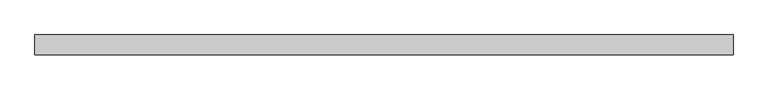
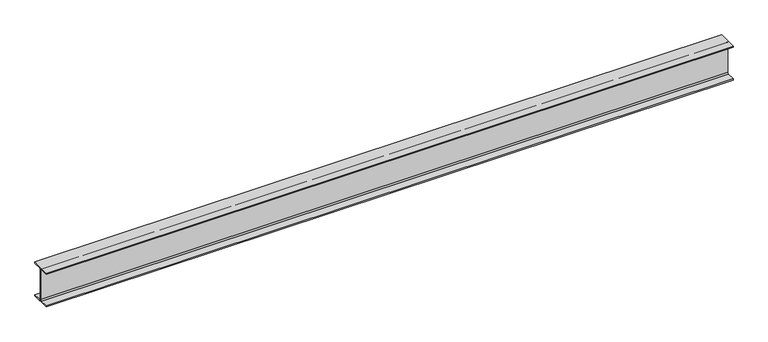
"""IFC4 building model written with IfcOpenShell, lengths in millimetres: beam geometry, Old_Steel Beam_H-KSD3502 : H_SB_ASB_H-350×175x7x11."""

import ifcopenshell
import ifcopenshell.guid

model = None  # the IFC model being written
_history = None  # IfcOwnerHistory: only IFC2X3 demands one
_inside = {}  # id of a spatial element -> (the spatial element, [elements in it])
_under = {}  # id of a project, library or spatial element -> (it, [spatial elements below it])
_declared = {}  # id of a project -> (the project, [libraries it declares])
_typed = {}  # id of a type object -> (the type object, [elements of that type])
_made_of = {}  # id of a material, layer set ... -> (it, [elements and type objects made of it])


def new_model(schema):
    """Start an empty IFC model of exactly this schema.

    Asked for "IFC4X3", IfcOpenShell would pick the latest addendum, in which some entities
    have other attributes; the version numbers below select the first issue.
    IFC2X3 requires an IfcOwnerHistory on every rooted entity: one is made here for all.
    """
    global model, _history
    if schema == "IFC4X3":
        model = ifcopenshell.file(schema_version=(4, 3, 0, 0))
    else:
        model = ifcopenshell.file(schema=schema)
    _inside.clear()
    _under.clear()
    _declared.clear()
    _typed.clear()
    _made_of.clear()
    _history = None
    if model.schema == "IFC2X3":
        org = make("IfcOrganization", Name="unknown")
        user = make(
            "IfcPersonAndOrganization",
            ThePerson=make("IfcPerson", FamilyName="unknown"),
            TheOrganization=org,
        )
        app = make(
            "IfcApplication",
            ApplicationDeveloper=org,
            Version="unknown",
            ApplicationFullName="unknown",
            ApplicationIdentifier="unknown",
        )
        _history = make(
            "IfcOwnerHistory",
            OwningUser=user,
            OwningApplication=app,
            ChangeAction="ADDED",
            CreationDate=0,
        )
    return model


def make(cls, **values):
    """One entity of the class cls with the attributes given. An attribute that is None is left unset."""
    return model.create_entity(
        cls, **{name: value for name, value in values.items() if value is not None}
    )


def rooted(cls, **values):
    """An entity with a GlobalId (a new one), such as an element, a storey or a relation."""
    return make(cls, GlobalId=ifcopenshell.guid.new(), OwnerHistory=_history, **values)


def si_unit(unit_type, name, prefix=None):
    """IfcSIUnit, for example si_unit("LENGTHUNIT", "METRE", prefix="MILLI")."""
    return make("IfcSIUnit", UnitType=unit_type, Prefix=prefix, Name=name)


def assignment(units):
    """IfcUnitAssignment: the units of a project."""
    return None if units is None else make("IfcUnitAssignment", Units=units)


def point(xyz):
    """IfcCartesianPoint."""
    return None if xyz is None else make("IfcCartesianPoint", Coordinates=xyz)


def direction(xyz):
    """IfcDirection."""
    return None if xyz is None else make("IfcDirection", DirectionRatios=xyz)


def frame(location, z_axis=None, x_axis=None):
    """IfcAxis2Placement3D, a coordinate frame: its origin and axes. An axis left out is left unset."""
    return make(
        "IfcAxis2Placement3D",
        Location=point(location),
        Axis=direction(z_axis),
        RefDirection=direction(x_axis),
    )


def frame_2d(location, x_axis=None):
    """IfcAxis2Placement2D, a coordinate frame in the plane: its origin and x axis."""
    return make(
        "IfcAxis2Placement2D", Location=point(location), RefDirection=direction(x_axis)
    )


def origin():
    """The frame at (0, 0, 0) with its axes left unset."""
    return frame((0.0, 0.0, 0.0))


def place(relative_to, where):
    """IfcLocalPlacement: puts the frame where relative to a parent placement (None: the world)."""
    return make(
        "IfcLocalPlacement", PlacementRelTo=relative_to, RelativePlacement=where
    )


def context(
    kind, dimensions, precision=None, world=None, true_north=None, identifier=None
):
    """IfcGeometricRepresentationContext, for example the 3D "Model" context."""
    return make(
        "IfcGeometricRepresentationContext",
        ContextIdentifier=identifier,
        ContextType=kind,
        CoordinateSpaceDimension=dimensions,
        Precision=precision,
        WorldCoordinateSystem=world,
        TrueNorth=true_north,
    )


def project(units=None, contexts=None):
    """IfcProject with its units and contexts."""
    return rooted(
        "IfcProject",
        Name="project",
        RepresentationContexts=contexts,
        UnitsInContext=assignment(units),
    )


def spatial(cls, under=None, at=None, **own):
    """A site, building, storey or space (cls), placed at a placement, below another one or the project."""
    s = rooted(cls, ObjectPlacement=at, **own)
    if under is not None:
        _under.setdefault(under.id(), (under, []))[1].append(s)
    return s


def polyline(points):
    """IfcPolyline through the points."""
    return make("IfcPolyline", Points=[point(p) for p in points])


def circle_curve(where, radius):
    """IfcCircle in the frame where."""
    return make("IfcCircle", Position=where, Radius=radius)


def trimmed(basis, trim1, trim2, sense, master):
    """IfcTrimmedCurve: the piece of a basis curve between two trims."""
    return make(
        "IfcTrimmedCurve",
        BasisCurve=basis,
        Trim1=trim1,
        Trim2=trim2,
        SenseAgreement=sense,
        MasterRepresentation=master,
    )


def segment(curve, same_sense, transition):
    """IfcCompositeCurveSegment."""
    return make(
        "IfcCompositeCurveSegment",
        Transition=transition,
        SameSense=same_sense,
        ParentCurve=curve,
    )


def composite_curve(segments, self_intersect=None):
    """IfcCompositeCurve: segments joined end to end."""
    return make("IfcCompositeCurve", Segments=segments, SelfIntersect=self_intersect)


def outline(outer, holes=None, kind="AREA"):
    """IfcArbitraryClosedProfileDef: a profile drawn as a closed curve; with holes, ...WithVoids."""
    if holes is None:
        return make("IfcArbitraryClosedProfileDef", ProfileType=kind, OuterCurve=outer)
    return make(
        "IfcArbitraryProfileDefWithVoids",
        ProfileType=kind,
        OuterCurve=outer,
        InnerCurves=holes,
    )


def extrude(swept, where, along, depth):
    """IfcExtrudedAreaSolid: the profile swept, set in the frame where, extruded along a direction by depth."""
    return make(
        "IfcExtrudedAreaSolid",
        SweptArea=swept,
        Position=where,
        ExtrudedDirection=direction(along),
        Depth=depth,
    )


def shape(context_of_items, identifier, shape_type, items):
    """IfcShapeRepresentation: the items that make up one representation, for example the "Body"."""
    return make(
        "IfcShapeRepresentation",
        ContextOfItems=context_of_items,
        RepresentationIdentifier=identifier,
        RepresentationType=shape_type,
        Items=items,
    )


def source(mapping_origin, context_of_items, identifier, shape_type, items):
    """IfcRepresentationMap: a shape defined once, which mapped items show again and again."""
    return make(
        "IfcRepresentationMap",
        MappingOrigin=mapping_origin,
        MappedRepresentation=shape(context_of_items, identifier, shape_type, items),
    )


def transform(
    local_origin,
    x_axis=None,
    y_axis=None,
    z_axis=None,
    scale=None,
    scale2=None,
    scale3=None,
    uniform=True,
):
    """IfcCartesianTransformationOperator3D, or its non-uniform kind. x_axis, y_axis, z_axis: its Axis1, 2, 3."""
    if uniform:
        return make(
            "IfcCartesianTransformationOperator3D",
            Axis1=direction(x_axis),
            Axis2=direction(y_axis),
            LocalOrigin=point(local_origin),
            Scale=scale,
            Axis3=direction(z_axis),
        )
    return make(
        "IfcCartesianTransformationOperator3DnonUniform",
        Axis1=direction(x_axis),
        Axis2=direction(y_axis),
        LocalOrigin=point(local_origin),
        Scale=scale,
        Axis3=direction(z_axis),
        Scale2=scale2,
        Scale3=scale3,
    )


def mapped(mapping_source, mapping_target):
    """IfcMappedItem: shows the shape of a source again, moved by a transform."""
    return make(
        "IfcMappedItem", MappingSource=mapping_source, MappingTarget=mapping_target
    )


def made_of(thing, what):
    """Note that an element or type object is made of a material, layer set ...; save() writes the relation."""
    if what is not None:
        _made_of.setdefault(what.id(), (what, []))[1].append(thing)
    return thing


def element(
    cls,
    number,
    at=None,
    inside=None,
    cuts=None,
    type_object=None,
    material=None,
    context=None,
    identifier="Body",
    shape_type=None,
    held_by="IfcProductDefinitionShape",
    body=None,
    shapes=None,
    **own,
):
    """One element of the class cls, such as IfcWall. Its Tag is "e" and its number.

    at: its placement. inside: the storey or other place that contains it. cuts: it is an
    opening in that element (IfcRelVoidsElement). A single representation is given by context,
    identifier, shape_type and body (its items); several are given by shapes. held_by: the class
    of the entity that holds the representations. save() writes the other relations.
    """
    e = rooted(cls, Tag="e%d" % number, ObjectPlacement=at, **own)
    if body is not None:
        shapes = [shape(context, identifier, shape_type, body)]
    if shapes is not None:
        e.Representation = make(held_by, Representations=shapes)
    if inside is not None:
        _inside.setdefault(inside.id(), (inside, []))[1].append(e)
    if cuts is not None:
        rooted(
            "IfcRelVoidsElement", RelatingBuildingElement=cuts, RelatedOpeningElement=e
        )
    if type_object is not None:
        _typed.setdefault(type_object.id(), (type_object, []))[1].append(e)
    return made_of(e, material)


def aggregate(whole, parts):
    """IfcRelAggregates: a whole, such as a stair, and the parts it consists of."""
    return rooted("IfcRelAggregates", RelatingObject=whole, RelatedObjects=parts)


def save(model, path):
    """Write the relations noted so far, then the file.

    IfcRelAggregates (storeys below a building ...), IfcRelContainedInSpatialStructure (elements
    in a storey), IfcRelDefinesByType, IfcRelAssociatesMaterial and IfcRelDeclares: one each for
    every whole, place, type object, material and project.
    """
    for whole, parts in _under.values():
        aggregate(whole, parts)
    for where, things in _inside.values():
        rooted(
            "IfcRelContainedInSpatialStructure",
            RelatedElements=things,
            RelatingStructure=where,
        )
    for kind, things in _typed.values():
        rooted("IfcRelDefinesByType", RelatedObjects=things, RelatingType=kind)
    for what, things in _made_of.values():
        rooted("IfcRelAssociatesMaterial", RelatedObjects=things, RelatingMaterial=what)
    for by, libraries in _declared.values():
        rooted("IfcRelDeclares", RelatingContext=by, RelatedDefinitions=libraries)
    model.write(path)


def beam_c0192abc(model_context):
    return source(origin(), model_context, "Body", "SweptSolid", [
        extrude(outline(composite_curve([segment(polyline([(82.5, -141.5), (82.5, -151.7), (-82.5, -151.7), (-82.5, -141.5), (-11.9, -141.5)]), True, "CONTINUOUS"), segment(trimmed(circle_curve(frame_2d((-11.9, -132.6)), 8.9), [point((-11.9, -141.5))], [point((-3.0, -132.6))], True, "CARTESIAN"), True, "CONTINUOUS"), segment(polyline([(-3.0, -132.6), (-3.0, 132.6)]), True, "CONTINUOUS"), segment(trimmed(circle_curve(frame_2d((-11.9, 132.6)), 8.9), [point((-3.0, 132.6))], [point((-11.9, 141.5))], True, "CARTESIAN"), True, "CONTINUOUS"), segment(polyline([(-11.9, 141.5), (-82.5, 141.5), (-82.5, 151.7), (82.5, 151.7), (82.5, 141.5), (11.9, 141.5)]), True, "CONTINUOUS"), segment(trimmed(circle_curve(frame_2d((11.9, 132.6)), 8.9), [point((11.9, 141.5))], [point((3.0, 132.6))], True, "CARTESIAN"), True, "CONTINUOUS"), segment(polyline([(3.0, 132.6), (3.0, -132.6)]), True, "CONTINUOUS"), segment(trimmed(circle_curve(frame_2d((11.9, -132.6)), 8.9), [point((3.0, -132.6))], [point((11.9, -141.5))], True, "CARTESIAN"), True, "CONTINUOUS"), segment(polyline([(11.9, -141.5), (82.5, -141.5)]), True, "CONTINUOUS")], self_intersect=False)), frame((-2914.177743, 0.0, 0.0), z_axis=(1.0, 0.0, 0.0), x_axis=(0.0, 1.0, 0.0)), (0.0, 0.0, 1.0), 5812.2452865),
    ])


if __name__ == "__main__":
    model = new_model("IFC4")
    model_context = context("Model", 3, world=origin())
    ifc_project = project(units=[si_unit("LENGTHUNIT", "METRE", prefix="MILLI")], contexts=[model_context])
    site = spatial("IfcSite", under=ifc_project)
    building = spatial("IfcBuilding", under=site)
    placement = place(None, origin())
    beam_shape = beam_c0192abc(model_context)
    element("IfcBeam", 1, ObjectType="Old_Steel Beam_H-KSD3502 : H_SB_ASB_H-350×175x7x11", at=placement, inside=building, context=model_context, shape_type="MappedRepresentation", body=[
        mapped(beam_shape, transform((0.0, 0.0, 0.0), x_axis=(1.0, 0.0, 0.0), y_axis=(0.0, 1.0, 0.0), z_axis=(0.0, 0.0, 1.0))),
    ])
    save(model, "model.ifc")

# Revit data of these elements
# Type "Old_Steel Beam_H-KSD3502 : H_SB_ASB_H-350×175x7x11"
#   Width = 17.5 cm
#   Web Thickness = 0.7 cm
#   Web Fillet = 1.4 cm
#   Warping Constant = 282290.0 cm⁶
#   Torsional Moment of Inertia = 19.4042 cm⁴
#   Torsional Modulus = 1.0 cm³
#   Section Area = 63.14 cm²
#   Plastic Modulus weak axis = 174.0 cm³
#   Plastic Modulus strong axis = 868.0 cm³
#   Perimeter = 1.36 m²/m
#   Nominal Weight = 49.60 kgf/m
#   Moment of Inertia weak axis = 984.00 cm⁴
#   Moment of Inertia strong axis = 13600.00 cm⁴
#   Height = 35.0 cm
#   Flange Thickness = 1.1 cm
#   Elastic Modulus weak axis = 112.0 cm³
#   Elastic Modulus strong axis = 775.0 cm³
#   Centroid Vertical = 17.5 cm
#   Centroid Horizontal = 8.75 cm
#   Length [instance default] = 1.5240 m
#   Structural Material [instance default] = Steel, 45-345
#   Assembly Code = ""
# Element 1 (IfcBeam, "Old_Steel Beam_H-KSD3502 : H_SB_ASB_H-350×175x7x11")
#   Structural Material = none
# Materials
#   "Steel, 45-345": class "Metal", colour RGB 189 187 185, transparency 0, Description = "Steel 345 MPa", Cost = 0
